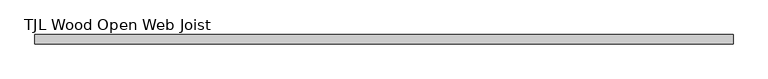
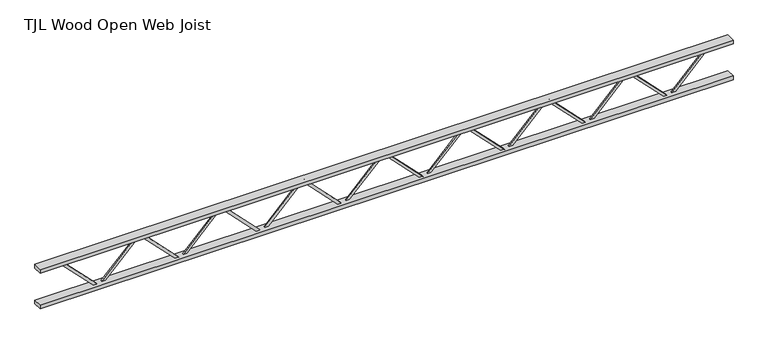
"""IFC4 building model written with IfcOpenShell, lengths in millimetres: beam geometry, TJL Wood Open Web Joist."""

from ifc_helpers import new_model, si_unit, frame, origin, place, context, project, spatial, polyline, outline, extrude, source, transform, mapped, element, save


def tjl_wood_open_web_joist_7ee492ce(model_context):
    return source(origin(), model_context, "Body", "SweptSolid", [
        extrude(outline(polyline([(171.45, 2384.2265625), (196.85, 2384.2265625), (196.85, 2366.1734945), (-171.45, 2006.9024007), (-171.45, 1961.4554688), (-196.85, 1961.4554688), (-196.85, 2017.6085368), (171.45, 2376.8796305), (171.45, 2384.2265625)])), frame((0.0, 0.0, 0.0), z_axis=(0.0, 1.0, 0.0), x_axis=(0.0, 0.0, 1.0)), (0.0, 0.0, 1.0), 12.7),
        extrude(outline(polyline([(196.85, 1589.484375), (171.45, 1589.484375), (171.45, 1596.831307), (-196.85, 1956.1024007), (-196.85, 2012.2554688), (-171.45, 2012.2554688), (-171.45, 1966.8085368), (196.85, 1607.537443), (196.85, 1589.484375)])), frame((0.0, -12.7, 0.0), z_axis=(0.0, 1.0, 0.0), x_axis=(0.0, 0.0, 1.0)), (0.0, 0.0, 1.0), 12.7),
        extrude(outline(polyline([(171.45, 1589.484375), (196.85, 1589.484375), (196.85, 1571.431307), (-171.45, 1212.1602132), (-171.45, 1166.7132813), (-196.85, 1166.7132813), (-196.85, 1222.8663493), (171.45, 1582.137443), (171.45, 1589.484375)])), frame((0.0, 0.0, 0.0), z_axis=(0.0, 1.0, 0.0), x_axis=(0.0, 0.0, 1.0)), (0.0, 0.0, 1.0), 12.7),
        extrude(outline(polyline([(196.85, 794.7421875), (171.45, 794.7421875), (171.45, 802.0891195), (-196.85, 1161.3602132), (-196.85, 1217.5132813), (-171.45, 1217.5132813), (-171.45, 1172.0663493), (196.85, 812.7952555), (196.85, 794.7421875)])), frame((0.0, -12.7, 0.0), z_axis=(0.0, 1.0, 0.0), x_axis=(0.0, 0.0, 1.0)), (0.0, 0.0, 1.0), 12.7),
        extrude(outline(polyline([(171.45, 794.7421875), (196.85, 794.7421875), (196.85, 776.6891195), (-171.45, 417.4180257), (-171.45, 371.9710938), (-196.85, 371.9710938), (-196.85, 428.1241618), (171.45, 787.3952555), (171.45, 794.7421875)])), frame((0.0, 0.0, 0.0), z_axis=(0.0, 1.0, 0.0), x_axis=(0.0, 0.0, 1.0)), (0.0, 0.0, 1.0), 12.7),
        extrude(outline(polyline([(196.85, 0.0), (171.45, 0.0), (171.45, 7.346932), (-196.85, 366.6180257), (-196.85, 422.7710938), (-171.45, 422.7710938), (-171.45, 377.3241618), (196.85, 18.053068), (196.85, 0.0)])), frame((0.0, -12.7, 0.0), z_axis=(0.0, 1.0, 0.0), x_axis=(0.0, 0.0, 1.0)), (0.0, 0.0, 1.0), 12.7),
        extrude(outline(polyline([(171.45, 0.0), (196.85, 0.0), (196.85, -18.053068), (-171.45, -377.3241618), (-171.45, -422.7710937), (-196.85, -422.7710937), (-196.85, -366.6180257), (171.45, -7.346932), (171.45, 0.0)])), frame((0.0, 0.0, 0.0), z_axis=(0.0, 1.0, 0.0), x_axis=(0.0, 0.0, 1.0)), (0.0, 0.0, 1.0), 12.7),
        extrude(outline(polyline([(196.85, -794.7421875), (171.45, -794.7421875), (171.45, -787.3952555), (-196.85, -428.1241618), (-196.85, -371.9710937), (-171.45, -371.9710937), (-171.45, -417.4180257), (196.85, -776.6891195), (196.85, -794.7421875)])), frame((0.0, -12.7, 0.0), z_axis=(0.0, 1.0, 0.0), x_axis=(0.0, 0.0, 1.0)), (0.0, 0.0, 1.0), 12.7),
        extrude(outline(polyline([(171.45, -794.7421875), (196.85, -794.7421875), (196.85, -812.7952555), (-171.45, -1172.0663493), (-171.45, -1217.5132812), (-196.85, -1217.5132812), (-196.85, -1161.3602132), (171.45, -802.0891195), (171.45, -794.7421875)])), frame((0.0, 0.0, 0.0), z_axis=(0.0, 1.0, 0.0), x_axis=(0.0, 0.0, 1.0)), (0.0, 0.0, 1.0), 12.7),
        extrude(outline(polyline([(196.85, -1589.484375), (171.45, -1589.484375), (171.45, -1582.137443), (-196.85, -1222.8663493), (-196.85, -1166.7132812), (-171.45, -1166.7132812), (-171.45, -1212.1602132), (196.85, -1571.431307), (196.85, -1589.484375)])), frame((0.0, -12.7, 0.0), z_axis=(0.0, 1.0, 0.0), x_axis=(0.0, 0.0, 1.0)), (0.0, 0.0, 1.0), 12.7),
        extrude(outline(polyline([(171.45, -1589.484375), (196.85, -1589.484375), (196.85, -1607.537443), (-171.45, -1966.8085368), (-171.45, -2012.2554687), (-196.85, -2012.2554687), (-196.85, -1956.1024007), (171.45, -1596.831307), (171.45, -1589.484375)])), frame((0.0, 0.0, 0.0), z_axis=(0.0, 1.0, 0.0), x_axis=(0.0, 0.0, 1.0)), (0.0, 0.0, 1.0), 12.7),
        extrude(outline(polyline([(196.85, -2384.2265625), (171.45, -2384.2265625), (171.45, -2376.8796305), (-196.85, -2017.6085368), (-196.85, -1961.4554687), (-171.45, -1961.4554687), (-171.45, -2006.9024007), (196.85, -2366.1734945), (196.85, -2384.2265625)])), frame((0.0, -12.7, 0.0), z_axis=(0.0, 1.0, 0.0), x_axis=(0.0, 0.0, 1.0)), (0.0, 0.0, 1.0), 12.7),
        extrude(outline(polyline([(171.45, 3178.96875), (196.85, 3178.96875), (196.85, 3160.915682), (-171.45, 2801.6445882), (-171.45, 2756.1976563), (-196.85, 2756.1976563), (-196.85, 2812.3507243), (171.45, 3171.621818), (171.45, 3178.96875)])), frame((0.0, 0.0, 0.0), z_axis=(0.0, 1.0, 0.0), x_axis=(0.0, 0.0, 1.0)), (0.0, 0.0, 1.0), 12.7),
        extrude(outline(polyline([(196.85, 2384.2265625), (171.45, 2384.2265625), (171.45, 2391.5734945), (-196.85, 2750.8445882), (-196.85, 2806.9976563), (-171.45, 2806.9976563), (-171.45, 2761.5507243), (196.85, 2402.2796305), (196.85, 2384.2265625)])), frame((0.0, -12.7, 0.0), z_axis=(0.0, 1.0, 0.0), x_axis=(0.0, 0.0, 1.0)), (0.0, 0.0, 1.0), 12.7),
        extrude(outline(polyline([(171.45, -2384.2265625), (196.85, -2384.2265625), (196.85, -2402.2796305), (-171.45, -2761.5507243), (-171.45, -2806.9976562), (-196.85, -2806.9976562), (-196.85, -2750.8445882), (171.45, -2391.5734945), (171.45, -2384.2265625)])), frame((0.0, 0.0, 0.0), z_axis=(0.0, 1.0, 0.0), x_axis=(0.0, 0.0, 1.0)), (0.0, 0.0, 1.0), 12.7),
        extrude(outline(polyline([(196.85, -3178.96875), (171.45, -3178.96875), (171.45, -3171.621818), (-196.85, -2812.3507243), (-196.85, -2756.1976562), (-171.45, -2756.1976562), (-171.45, -2801.6445882), (196.85, -3160.915682), (196.85, -3178.96875)])), frame((0.0, -12.7, 0.0), z_axis=(0.0, 1.0, 0.0), x_axis=(0.0, 0.0, 1.0)), (0.0, 0.0, 1.0), 12.7),
        extrude(outline(polyline([(3382.16875, 44.45), (3382.16875, -44.45), (-3382.16875, -44.45), (-3382.16875, 44.45), (3382.16875, 44.45)])), frame((0.0, 0.0, 165.1), z_axis=(0.0, 0.0, 1.0), x_axis=(1.0, 0.0, 0.0)), (0.0, 0.0, 1.0), 38.1),
        extrude(outline(polyline([(3382.16875, 44.45), (3382.16875, -44.45), (-3382.16875, -44.45), (-3382.16875, 44.45), (3382.16875, 44.45)])), frame((0.0, 0.0, -203.2), z_axis=(0.0, 0.0, 1.0), x_axis=(1.0, 0.0, 0.0)), (0.0, 0.0, 1.0), 38.1),
    ])


if __name__ == "__main__":
    model = new_model("IFC4")
    model_context = context("Model", 3, world=origin())
    ifc_project = project(units=[si_unit("LENGTHUNIT", "METRE", prefix="MILLI")], contexts=[model_context])
    site = spatial("IfcSite", under=ifc_project)
    building = spatial("IfcBuilding", under=site)
    placement = place(None, origin())
    tjl_wood_open_web_joist_shape = tjl_wood_open_web_joist_7ee492ce(model_context)
    element("IfcBeam", 1, ObjectType="TJL Wood Open Web Joist : 16\" PREENGINEERED FLOOR TRUSS", at=placement, inside=building, context=model_context, shape_type="MappedRepresentation", body=[
        mapped(tjl_wood_open_web_joist_shape, transform((0.0, 0.0, 0.0), x_axis=(1.0, 0.0, 0.0), y_axis=(0.0, 1.0, 0.0), z_axis=(0.0, 0.0, 1.0))),
    ])
    save(model, "model.ifc")

# Revit data of these elements
# Type "TJL Wood Open Web Joist : 16\" PREENGINEERED FLOOR TRUSS"
#   Web Thickness = 0' - 1"
#   Web Leg = 0' - 1"
#   Start Offset [instance default] = 0' - 0"
#   Top Chord Start Extension [instance default] = 0' - 0"
#   PanelArrayLength [instance default] = 22' - 8"
#   Depth = 1' - 4"
#   PanelWidth [instance default] = 2' - 6.22222"
#   Offset Length 2 [instance default] = 0' - 8"
#   Offset Length 1 [instance default] = 0' - 8"
#   End Panel [instance default] = 0' - 8"
#   End Offset [instance default] = 0' - 0"
#   Top Chord End Extension [instance default] = 0' - 0"
#   Chord Width = 0' - 3 1/2"
#   Chord Depth = 0' - 1 1/2"
#   Bottom Chord Start Extension [instance default] = 0' - 0"
#   Bottom Chord End Extension [instance default] = 0' - 0"
#   Length [instance default] = 24' - 0"
#   PanelArrayNum [instance default] = 9
#   Web Rendering Material = none
#   Structural Material = none
#   Assembly Code = ""
# Element 1 (IfcBeam, "TJL Wood Open Web Joist : 16\" PREENGINEERED FLOOR TRUSS")
#   PanelArrayLength = 20' - 10 5/16"
#   PanelWidth = 2' - 7 37/128"
#   PanelArrayNum = 8
